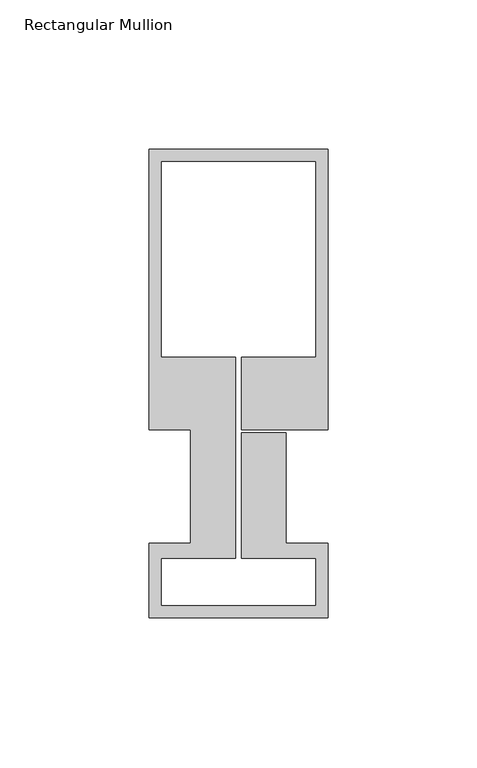
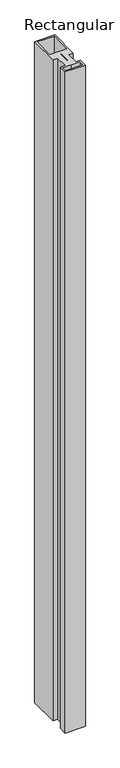
"""IFC4 building model written with IfcOpenShell, lengths in millimetres: member geometry, Rectangular Mullion : Schueco_FWS-60-SI_Mull_CovCap-20mm_Mull-85mm."""

from ifc_helpers import new_model, si_unit, frame, origin, place, context, project, spatial, polyline, outline, extrude, source, transform, mapped, element, save


def rectangular_mullion_659b9bea(model_context):
    return source(origin(), model_context, "Body", "SweptSolid", [
        extrude(outline(polyline([(-60.0, 132.0), (0.0, 132.0), (0.0, 38.0), (-29.0, 38.0), (-29.0, 62.3), (-4.0, 62.3), (-4.0, 128.0), (-56.0, 128.0), (-56.0, 62.3), (-31.0, 62.3), (-31.0, -5.0), (-56.0, -5.0), (-56.0, -21.0), (-4.0, -21.0), (-4.0, -5.0), (-29.0, -5.0), (-29.0, 37.0), (-14.0, 37.0), (-14.0, -0.1), (0.0, -0.1), (0.0, -25.0), (-60.0, -25.0), (-60.0, -0.1), (-46.0, -0.1), (-46.0, 38.0), (-60.0, 38.0), (-60.0, 132.0)])), frame((0.0, 0.0, -2080.0), z_axis=(0.0, 0.0, 1.0), x_axis=(1.0, 0.0, 0.0)), (0.0, 0.0, 1.0), 2080.0),
    ])


if __name__ == "__main__":
    model = new_model("IFC4")
    model_context = context("Model", 3, world=origin())
    ifc_project = project(units=[si_unit("LENGTHUNIT", "METRE", prefix="MILLI")], contexts=[model_context])
    site = spatial("IfcSite", under=ifc_project)
    building = spatial("IfcBuilding", under=site)
    placement = place(None, origin())
    rectangular_mullion_shape = rectangular_mullion_659b9bea(model_context)
    element("IfcMember", 1, ObjectType="Rectangular Mullion : Schueco_FWS-60-SI_Mull_CovCap-20mm_Mull-85mm", at=placement, inside=building, context=model_context, shape_type="MappedRepresentation", body=[
        mapped(rectangular_mullion_shape, transform((0.0, 0.0, 0.0), x_axis=(1.0, 0.0, 0.0), y_axis=(0.0, 1.0, 0.0), z_axis=(0.0, 0.0, 1.0))),
    ])
    save(model, "model.ifc")

# Revit data of these elements
# Type "Rectangular Mullion : Schueco_FWS-60-SI_Mull_CovCap-20mm_Mull-85mm"
#   Model = "FWS 60.SI"
#   Manufacturer = "Schueco International KG"
#   Type Comments = "Mullion"
#   Schueco thermal insulation standard = "Suitable for passive houses"
#   Burglar resistance = "RC 3"
#   Thermal insulation = "to 0.70 W/(m²K)"
#   built-in parameter 1007322 = 0.515092 (stored number, unit not read)
#   built-in parameter 1007321 = 0.0524934 (stored number, unit not read)
#   built-in parameter 1007320 = 0.0524934 (stored number, unit not read)
# Element 1 (IfcMember, "Rectangular Mullion : Schueco_FWS-60-SI_Mull_CovCap-20mm_Mull-85mm")
#   Materials on its faces: "Alu"
# Materials
#   "Alu": class "Glas", colour RGB 140 140 140, transparency 0
